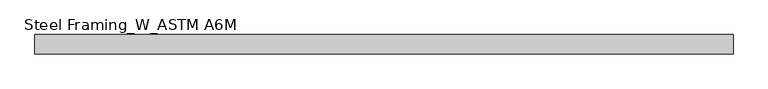
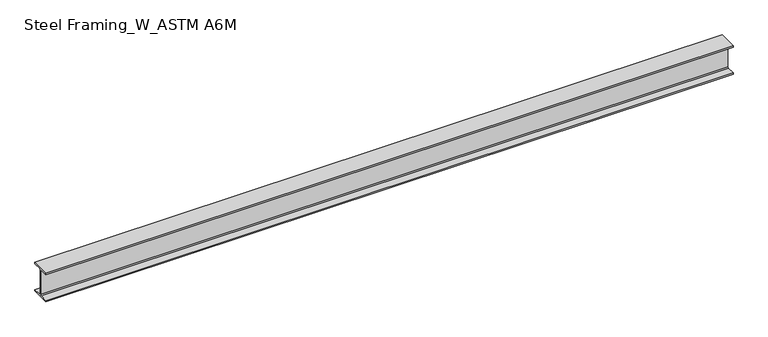
"""IFC4 building model written with IfcOpenShell, lengths in millimetres: beam geometry, Steel Framing_W_ASTM A6M : H_SB_AR_S02_W200x31.3_RB4."""

from ifc_helpers import new_model, si_unit, point, frame, frame_2d, origin, place, context, project, spatial, polyline, circle_curve, trimmed, segment, composite_curve, outline, extrude, source, transform, mapped, element, save


def steel_framing_w_astm_a6m_505f7bb4(model_context):
    return source(origin(), model_context, "Body", "SweptSolid", [
        extrude(outline(composite_curve([segment(polyline([(67.0, -94.8), (67.0, -105.0), (-67.0, -105.0), (-67.0, -94.8), (-10.775, -94.8)]), True, "CONTINUOUS"), segment(trimmed(circle_curve(frame_2d((-10.775, -87.2)), 7.6), [point((-10.775, -94.8))], [point((-3.175, -87.2))], True, "CARTESIAN"), True, "CONTINUOUS"), segment(polyline([(-3.175, -87.2), (-3.175, 87.2)]), True, "CONTINUOUS"), segment(trimmed(circle_curve(frame_2d((-10.775, 87.2)), 7.6), [point((-3.175, 87.2))], [point((-10.775, 94.8))], True, "CARTESIAN"), True, "CONTINUOUS"), segment(polyline([(-10.775, 94.8), (-67.0, 94.8), (-67.0, 105.0), (67.0, 105.0), (67.0, 94.8), (10.775, 94.8)]), True, "CONTINUOUS"), segment(trimmed(circle_curve(frame_2d((10.775, 87.2)), 7.6), [point((10.775, 94.8))], [point((3.175, 87.2))], True, "CARTESIAN"), True, "CONTINUOUS"), segment(polyline([(3.175, 87.2), (3.175, -87.2)]), True, "CONTINUOUS"), segment(trimmed(circle_curve(frame_2d((10.775, -87.2)), 7.6), [point((3.175, -87.2))], [point((10.775, -94.8))], True, "CARTESIAN"), True, "CONTINUOUS"), segment(polyline([(10.775, -94.8), (67.0, -94.8)]), True, "CONTINUOUS")], self_intersect=False)), frame((-2349.9, 0.0, 0.0), z_axis=(1.0, 0.0, 0.0), x_axis=(0.0, 1.0, 0.0)), (0.0, 0.0, 1.0), 4799.9),
    ])


if __name__ == "__main__":
    model = new_model("IFC4")
    model_context = context("Model", 3, world=origin())
    ifc_project = project(units=[si_unit("LENGTHUNIT", "METRE", prefix="MILLI")], contexts=[model_context])
    site = spatial("IfcSite", under=ifc_project)
    building = spatial("IfcBuilding", under=site)
    placement = place(None, origin())
    steel_framing_w_astm_a6m_shape = steel_framing_w_astm_a6m_505f7bb4(model_context)
    element("IfcBeam", 1, ObjectType="Steel Framing_W_ASTM A6M : H_SB_AR_S02_W200x31.3_RB4", at=placement, inside=building, context=model_context, shape_type="MappedRepresentation", body=[
        mapped(steel_framing_w_astm_a6m_shape, transform((0.0, 0.0, 0.0), x_axis=(1.0, 0.0, 0.0), y_axis=(0.0, 1.0, 0.0), z_axis=(0.0, 0.0, 1.0))),
    ])
    save(model, "model.ifc")

# Revit data of these elements
# Type "Steel Framing_W_ASTM A6M : H_SB_AR_S02_W200x31.3_RB4"
#   Type Mark = "RB4"
#   Section Name Key = "W8x21"
#   Width = 13.4 cm
#   Web Thickness = 0.635 cm
#   Web Fillet = 0.76 cm
#   Warping Constant = 40800.0 cm⁶
#   Torsional Moment of Inertia = 11.70 cm⁴
#   Section Area = 39.7 cm²
#   Plastic Modulus weak axis = 93.2 cm³
#   Plastic Modulus strong axis = 334.0 cm³
#   Perimeter = 0.93 m²/m
#   Nominal Weight = 31.30 kgf/m
#   Moment of Inertia weak axis = 407.00 cm⁴
#   Moment of Inertia strong axis = 3130.00 cm⁴
#   Height = 21.0 cm
#   Flange Thickness = 1.02 cm
#   Elastic Modulus weak axis = 60.8 cm³
#   Elastic Modulus strong axis = 298.0 cm³
#   Centroid Vertical = 10.5 cm
#   Centroid Horizontal = 6.7 cm
#   Length [instance default] = 1500 mm
#   Structural Material [instance default] = Steel, 45-345
#   Bolt Spacing = 0
#   Assembly Code = ""
# Element 1 (IfcBeam, "Steel Framing_W_ASTM A6M : H_SB_AR_S02_W200x31.3_RB4")
#   Materials on its faces: "Steel, 45-345"
# Materials
#   "Steel, 45-345": class "Metal", colour RGB 189 187 185, transparency 0, Description = "Steel 345 MPa", Cost = 0
